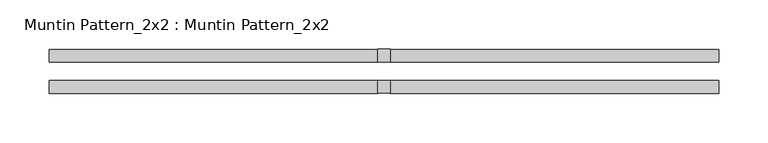
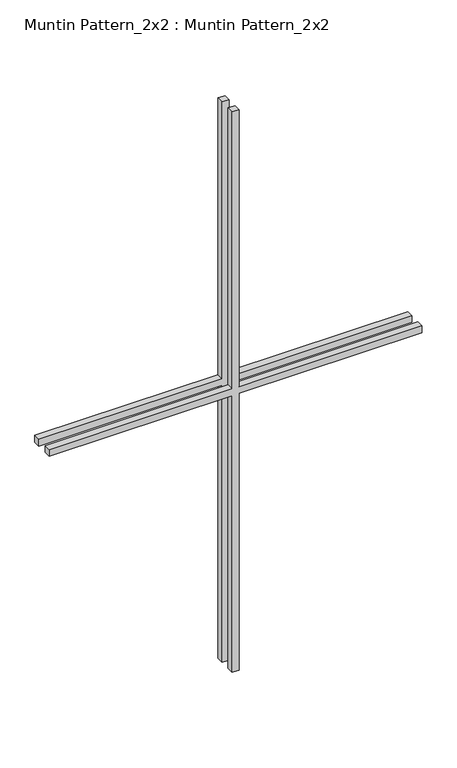
"""IFC4 building model written with IfcOpenShell, lengths in millimetres: proxy geometry, Muntin Pattern_2x2 : Muntin Pattern_2x2."""

from ifc_helpers import new_model, si_unit, frame, origin, place, context, project, spatial, polyline, outline, extrude, source, transform, mapped, element, save


def muntin_pattern_2x2_muntin_pattern_2x2_ec25664a(model_context):
    return source(origin(), model_context, "Body", "SweptSolid", [
        extrude(outline(polyline([(542.925, -6.35), (542.925, -338.1375), (530.225, -338.1375), (530.225, -6.35), (0.0, -6.35), (0.0, 6.35), (530.225, 6.35), (530.225, 338.1375), (542.925, 338.1375), (542.925, 6.35), (1073.15, 6.35), (1073.15, -6.35), (542.925, -6.35)])), frame((0.0, -22.225, 0.0), z_axis=(0.0, 1.0, 0.0), x_axis=(0.0, 0.0, 1.0)), (0.0, 0.0, 1.0), 12.7),
        extrude(outline(polyline([(542.925, -6.35), (542.925, -338.1375), (530.225, -338.1375), (530.225, -6.35), (0.0, -6.35), (0.0, 6.35), (530.225, 6.35), (530.225, 338.1375), (542.925, 338.1375), (542.925, 6.35), (1073.15, 6.35), (1073.15, -6.35), (542.925, -6.35)])), frame((0.0, 9.525, 0.0), z_axis=(0.0, 1.0, 0.0), x_axis=(0.0, 0.0, 1.0)), (0.0, 0.0, 1.0), 12.7),
    ])


if __name__ == "__main__":
    model = new_model("IFC4")
    model_context = context("Model", 3, world=origin())
    ifc_project = project(units=[si_unit("LENGTHUNIT", "METRE", prefix="MILLI")], contexts=[model_context])
    site = spatial("IfcSite", under=ifc_project)
    building = spatial("IfcBuilding", under=site)
    placement = place(None, origin())
    muntin_pattern_2x2_muntin_pattern_2x2_shape = muntin_pattern_2x2_muntin_pattern_2x2_ec25664a(model_context)
    element("IfcBuildingElementProxy", 1, Name="Muntin Pattern_2x2 : Muntin Pattern_2x2", ObjectType="Muntin Pattern_2x2 : Muntin Pattern_2x2", at=placement, inside=building, context=model_context, shape_type="MappedRepresentation", body=[
        mapped(muntin_pattern_2x2_muntin_pattern_2x2_shape, transform((0.0, 0.0, 0.0), x_axis=(1.0, 0.0, 0.0), y_axis=(0.0, 1.0, 0.0), z_axis=(0.0, 0.0, 1.0))),
    ])
    save(model, "model.ifc")

# Revit data of these elements
# Type "Muntin Pattern_2x2 : Muntin Pattern_2x2"
#   Width [instance default] = 4' - 0"
#   Thickness = 0' - 0 1/2"
#   Height [instance default] = 4' - 0"
#   Distance = 0' - 0 3/4"
#   Interior Material [instance default] = none
#   Exterior Material [instance default] = none
#   Default Elevation = 0
# Element 1 (IfcBuildingElementProxy, "Muntin Pattern_2x2 : Muntin Pattern_2x2")
#   Width = 2' - 2 5/8"
#   Height = 3' - 6 1/4"
#   Interior Material = Cherry
#   Exterior Material = PVC, Flexible
#   Materials on its faces: "PVC, Flexible", "Cherry"
# Materials
#   "PVC, Flexible": class "Plastic", colour RGB 178 178 178, transparency 0, Description = "Flexible polyvinyl chloride", Cost = 0
#   "Cherry": class "Wood", colour RGB 157 77 38, transparency 0, Description = "Prunus Serotina", Cost = 0
